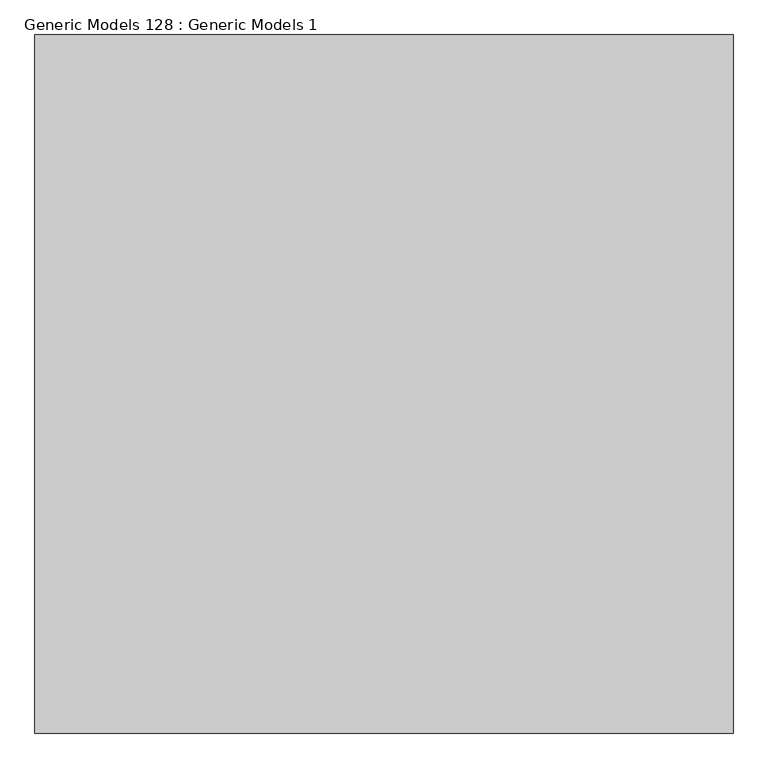
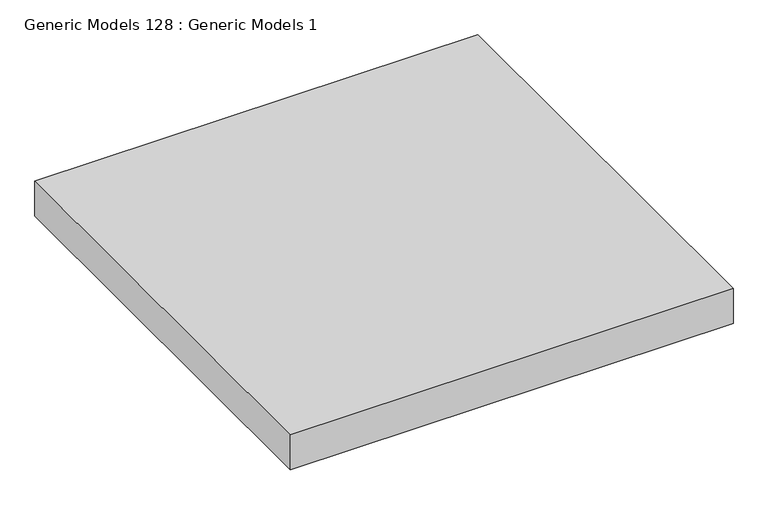
"""IFC4 building model written with IfcOpenShell, lengths in millimetres: proxy geometry, Generic Models 128 : Generic Models 1."""

from ifc_helpers import new_model, si_unit, frame, origin, place, context, project, spatial, polyline, outline, extrude, source, transform, mapped, element, save


def generic_models_128_generic_models_1_9921986f(model_context):
    return source(origin(), model_context, "Body", "SweptSolid", [
        extrude(outline(polyline([(47499.4360531, 0.0), (46280.2360531, 0.0), (46280.2360531, 1219.2), (47499.4360531, 1219.2), (47499.4360531, 0.0)])), frame((0.0, 0.0, 2231.473933), z_axis=(0.0, 0.0, 1.0), x_axis=(1.0, 0.0, 0.0)), (0.0, 0.0, 1.0), 101.6),
    ])


if __name__ == "__main__":
    model = new_model("IFC4")
    model_context = context("Model", 3, world=origin())
    ifc_project = project(units=[si_unit("LENGTHUNIT", "METRE", prefix="MILLI")], contexts=[model_context])
    site = spatial("IfcSite", under=ifc_project)
    building = spatial("IfcBuilding", under=site)
    placement = place(None, origin())
    generic_models_128_generic_models_1_shape = generic_models_128_generic_models_1_9921986f(model_context)
    element("IfcBuildingElementProxy", 1, Name="Generic Models 128 : Generic Models 1", ObjectType="Generic Models 128 : Generic Models 1", at=placement, inside=building, context=model_context, shape_type="MappedRepresentation", body=[
        mapped(generic_models_128_generic_models_1_shape, transform((0.0, 0.0, 0.0), x_axis=(1.0, 0.0, 0.0), y_axis=(0.0, 1.0, 0.0), z_axis=(0.0, 0.0, 1.0))),
    ])
    save(model, "model.ifc")

# Revit data of these elements
# Element 1 (IfcBuildingElementProxy, "Generic Models 128 : Generic Models 1")
#   Materials on its faces: "UNDERSIDE OF STRUCTURE"
# Materials
#   "UNDERSIDE OF STRUCTURE": class "Concrete", colour RGB 36 37 33, transparency 0, Description = "Lightweight concrete", Cost = 0
